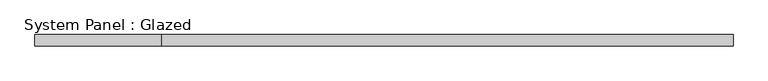
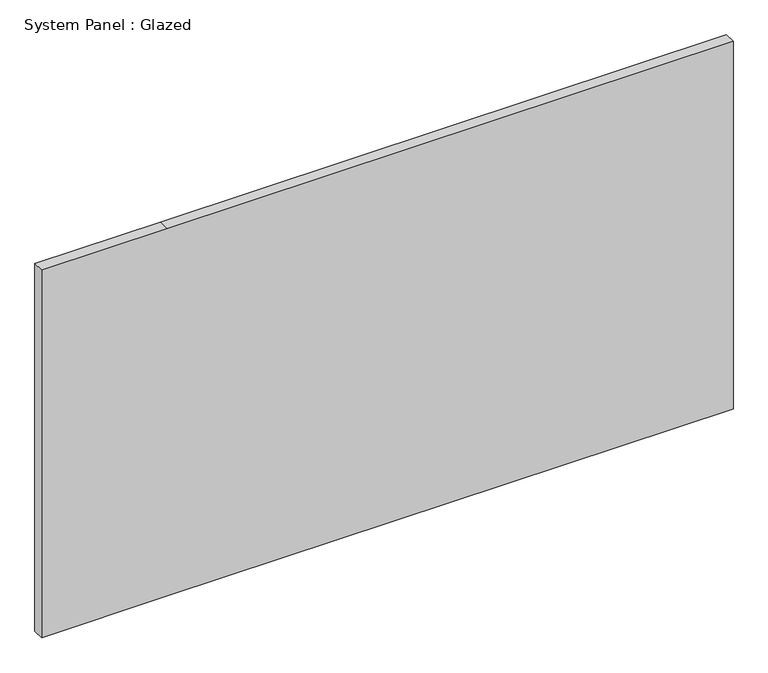
"""IFC4 building model written with IfcOpenShell, lengths in millimetres: plate geometry, System Panel : Glazed."""

from ifc_helpers import new_model, si_unit, frame, origin, place, context, project, spatial, polyline, outline, extrude, source, transform, mapped, element, save


def system_panel_glazed_9909c948(model_context):
    return source(origin(), model_context, "Body", "SweptSolid", [
        extrude(outline(polyline([(0.0, -768.35), (0.0, -488.95), (0.0, 768.35), (863.6, 768.35), (863.6, -488.95), (863.6, -768.35), (0.0, -768.35)])), frame((0.0, -44.45, 0.0), z_axis=(0.0, 1.0, 0.0), x_axis=(0.0, 0.0, 1.0)), (0.0, 0.0, 1.0), 25.4),
    ])


if __name__ == "__main__":
    model = new_model("IFC4")
    model_context = context("Model", 3, world=origin())
    ifc_project = project(units=[si_unit("LENGTHUNIT", "METRE", prefix="MILLI")], contexts=[model_context])
    site = spatial("IfcSite", under=ifc_project)
    building = spatial("IfcBuilding", under=site)
    placement = place(None, origin())
    system_panel_glazed_shape = system_panel_glazed_9909c948(model_context)
    element("IfcPlate", 1, ObjectType="System Panel : Glazed", at=placement, inside=building, context=model_context, shape_type="MappedRepresentation", body=[
        mapped(system_panel_glazed_shape, transform((0.0, 0.0, 0.0), x_axis=(1.0, 0.0, 0.0), y_axis=(0.0, 1.0, 0.0), z_axis=(0.0, 0.0, 1.0))),
    ])
    save(model, "model.ifc")

# Revit data of these elements
# Element 1 (IfcPlate, "System Panel : Glazed")
#   Materials on its faces: "Glass"
# Materials
#   "Glass": class "Glass", colour RGB 0 128 192, transparency 0.75, Cost = 0
